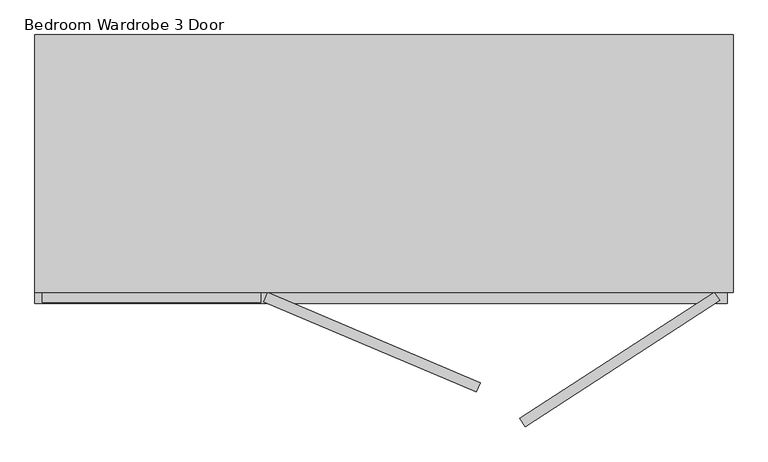
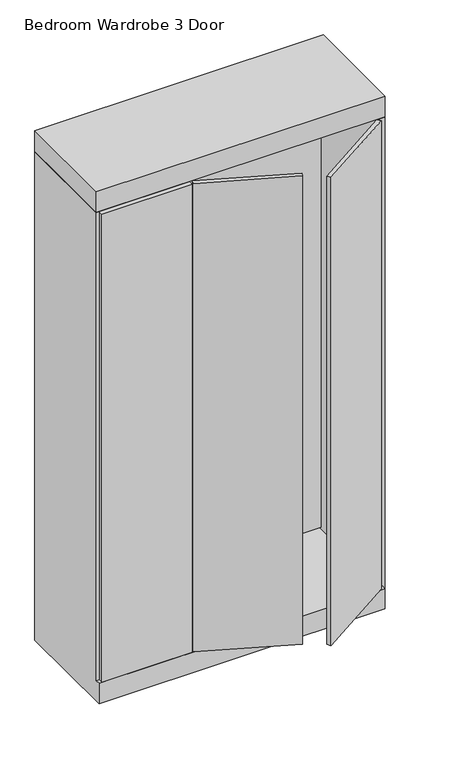
"""IFC4 building model written with IfcOpenShell, lengths in millimetres: furniture geometry, Bedroom Wardrobe 3 Door : Wardrobe 1300w x 550d x 2400h."""

from ifc_helpers import new_model, si_unit, frame, origin, place, context, project, spatial, polyline, outline, extrude, faceted_brep, source, transform, mapped, element, save


def bedroom_wardrobe_3_door_29ed634a(model_context):
    return source(origin(), model_context, "Body", "SolidModel", [
        extrude(outline(polyline([(338.8274532, -299.1040904), (-63.5175473, -128.3187703), (-56.0741193, -110.7831528), (346.2708812, -281.568473), (338.8274532, -299.1040904)])), frame((0.0, 0.0, 111.125), z_axis=(0.0, 0.0, 1.0), x_axis=(1.0, 0.0, 0.0)), (0.0, 0.0, 1.0), 2263.775),
        extrude(outline(polyline([(798.9376868, -125.9517987), (431.030381, -364.8735967), (420.6550073, -348.8969224), (788.5623132, -109.9751244), (798.9376868, -125.9517987)])), frame((0.0, 0.0, 111.125), z_axis=(0.0, 0.0, 1.0), x_axis=(1.0, 0.0, 0.0)), (0.0, 0.0, 1.0), 2263.775),
        extrude(outline(polyline([(-69.3208333, -129.0759615), (-482.6, -129.0759615), (-482.6, -110.0259615), (-69.3208333, -110.0259615), (-69.3208333, -129.0759615)])), frame((0.0, 0.0, 111.125), z_axis=(0.0, 0.0, 1.0), x_axis=(1.0, 0.0, 0.0)), (0.0, 0.0, 1.0), 2263.775),
        faceted_brep([(-471.0843944, -110.0894509, 2374.9), (-496.4843944, -110.0894509, 2374.9), (-496.4843944, -110.0894509, 111.125), (-471.0843944, -110.0894509, 111.125), (824.3156056, -110.0894509, 26.9875), (824.3156056, -110.0894509, 2374.9), (798.9156056, -110.0894509, 2374.9), (798.9156056, -110.0894509, 111.125), (812.8, -110.0894509, 111.125), (812.8, -110.0894509, 26.9875), (824.3156056, 377.3365385, 2374.9), (824.3156056, 377.3365385, 26.9875), (812.8, 377.3365385, 26.9875), (812.8, 377.3365385, 12.7), (-496.4843944, 377.3365385, 12.7), (-496.4843944, 377.3365385, 2374.9), (-471.0843944, 377.3365385, 120.65), (-471.0843944, 377.3365385, 111.125), (798.9156056, 377.3365385, 111.125), (798.9156056, 377.3365385, 120.65), (-471.0843944, 351.9365385, 2374.9), (798.9156056, 351.9365385, 2374.9), (-496.4843944, -130.6634615, 12.7), (-496.4843944, -130.6634615, 111.125), (-471.0843944, 351.9365385, 120.65), (798.9156056, 351.9365385, 120.65), (812.8, -130.6634615, 12.7), (812.8, -130.6634615, 111.125)], [[[0, 1, 2, 3]], [[4, 5, 6, 7, 8, 9]], [[10, 11, 12, 13, 14, 15], [16, 17, 18, 19]], [[1, 0, 20, 21, 6, 5, 10, 15]], [[1, 15, 14, 22, 23, 2]], [[20, 0, 3, 17, 16, 24]], [[11, 4, 9, 12]], [[5, 4, 11, 10]], [[6, 21, 25, 19, 18, 7]], [[21, 20, 24, 25]], [[16, 19, 25, 24]], [[26, 13, 12, 9, 8, 27]], [[13, 26, 22, 14]], [[23, 27, 8, 7, 18, 17, 3, 2]], [[26, 27, 23, 22]]]),
        faceted_brep([(824.3156056, -110.0894509, 2376.4093197), (824.3156056, -110.0894509, 2476.5), (-496.4843944, -110.0894509, 2476.5), (-496.4843944, -110.0894509, 2376.4093197), (824.3156056, 377.3365385, 2376.4093197), (-496.4843944, 377.3365385, 2376.4093197), (-496.4843944, 377.3365385, 2476.5), (824.3156056, 377.3365385, 2476.5)], [[[0, 1, 2, 3]], [[4, 5, 6, 7]], [[1, 0, 4, 7]], [[2, 1, 7, 6]], [[3, 2, 6, 5]], [[0, 3, 5, 4]]]),
    ])


if __name__ == "__main__":
    model = new_model("IFC4")
    model_context = context("Model", 3, world=origin())
    ifc_project = project(units=[si_unit("LENGTHUNIT", "METRE", prefix="MILLI")], contexts=[model_context])
    site = spatial("IfcSite", under=ifc_project)
    building = spatial("IfcBuilding", under=site)
    placement = place(None, origin())
    bedroom_wardrobe_3_door_shape = bedroom_wardrobe_3_door_29ed634a(model_context)
    element("IfcFurniture", 1, ObjectType="Bedroom Wardrobe 3 Door : Wardrobe 1300w x 550d x 2400h", at=placement, inside=building, context=model_context, shape_type="MappedRepresentation", body=[
        mapped(bedroom_wardrobe_3_door_shape, transform((0.0, 0.0, 0.0), x_axis=(1.0, 0.0, 0.0), y_axis=(0.0, 1.0, 0.0), z_axis=(0.0, 0.0, 1.0))),
    ])
    save(model, "model.ifc")

# Revit data of these elements
# Type "Bedroom Wardrobe 3 Door : Wardrobe 1300w x 550d x 2400h"
#   URL = "www.coalesse.com"
#   Type Comments = "CODWS5268"
#   Model = "Live/Work - Denizen"
#   Manufacturer = "Coalesse"
#   Description = "Wardobe Storage Tower"
#   Width = 1320.8 mm
#   Skirting = 101.6 mm
#   Pelmet = 101.6 mm
#   Height = 2438.4 mm
#   Depth = 508 mm
#   Cost = 5253
#   Hidden Right Leg = yes
#   Hidden Left Leg = yes
#   Frame = Wood - Walnut, Natural
#   Encasement = Wood - Walnut, Natural
#   Door Panel = Wood - Mahogany
# Element 1 (IfcFurniture, "Bedroom Wardrobe 3 Door : Wardrobe 1300w x 550d x 2400h")
#   Materials on its faces: "Wood - Mahogany", "Wood - Walnut, Natural"
# Materials
#   "Wood - Walnut, Natural": class "Wood", colour RGB 122 82 53, transparency 0
#   "Wood - Mahogany": class "Wood", colour RGB 138 86 45, transparency 0
